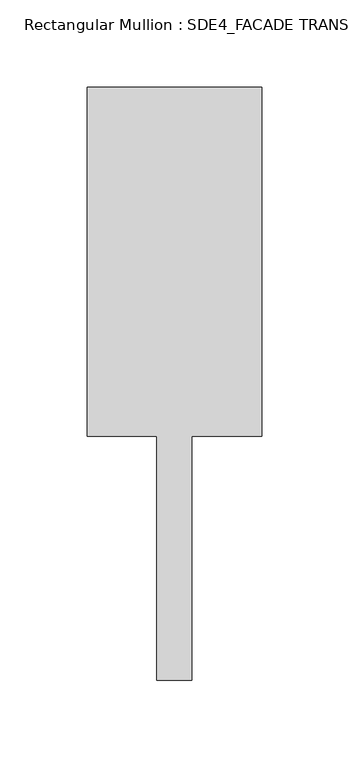
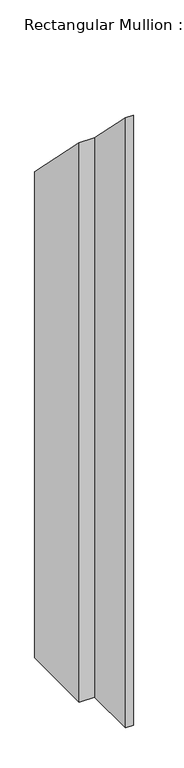
"""IFC4 building model written with IfcOpenShell, lengths in millimetres: member geometry, Rectangular Mullion : SDE4_FACADE TRANSOM TYPE 1."""

from ifc_helpers import new_model, si_unit, origin, place, context, project, spatial, faceted_brep, source, transform, mapped, element, save


def rectangular_mullion_sde4_facade_transom_type_1_69ea30fb(model_context):
    return source(origin(), model_context, "Body", "Brep", [
        faceted_brep([(50.0, 132.5, -1466.4475465), (50.0, -67.5, -1466.4475465), (10.0, -67.5, -1466.4475465), (10.0, -207.5, -1466.4475465), (-10.0, -207.5, -1466.4475465), (-10.0, -67.5, -1466.4475465), (-50.0, -67.5, -1466.4475465), (-50.0, 132.5, -1466.4475465), (-50.0, 132.5, -132.5), (50.0, 132.5, -132.5), (-50.0, -67.5, 67.5), (-10.0, -67.5, 67.5), (-10.0, -207.5, 207.5), (10.0, -207.5, 207.5), (10.0, -67.5, 67.5), (50.0, -67.5, 67.5)], [[[0, 1, 2, 3, 4, 5, 6, 7]], [[8, 9, 0, 7]], [[10, 8, 7, 6]], [[11, 10, 6, 5]], [[12, 11, 5, 4]], [[13, 12, 4, 3]], [[14, 13, 3, 2]], [[15, 14, 2, 1]], [[9, 15, 1, 0]], [[9, 8, 10, 11, 12, 13, 14, 15]]]),
    ])


if __name__ == "__main__":
    model = new_model("IFC4")
    model_context = context("Model", 3, world=origin())
    ifc_project = project(units=[si_unit("LENGTHUNIT", "METRE", prefix="MILLI")], contexts=[model_context])
    site = spatial("IfcSite", under=ifc_project)
    building = spatial("IfcBuilding", under=site)
    placement = place(None, origin())
    rectangular_mullion_sde4_facade_transom_type_1_shape = rectangular_mullion_sde4_facade_transom_type_1_69ea30fb(model_context)
    element("IfcMember", 1, ObjectType="Rectangular Mullion : SDE4_FACADE TRANSOM TYPE 1", at=placement, inside=building, context=model_context, shape_type="MappedRepresentation", body=[
        mapped(rectangular_mullion_sde4_facade_transom_type_1_shape, transform((0.0, 0.0, 0.0), x_axis=(1.0, 0.0, 0.0), y_axis=(0.0, 1.0, 0.0), z_axis=(0.0, 0.0, 1.0))),
    ])
    save(model, "model.ifc")

# Revit data of these elements
# Type "Rectangular Mullion : SDE4_FACADE TRANSOM TYPE 1"
#   built-in parameter 1007322 = 1.11549 (stored number, unit not read)
#   built-in parameter 1007321 = 0.164042 (stored number, unit not read)
#   built-in parameter 1007320 = 0.164042 (stored number, unit not read)
